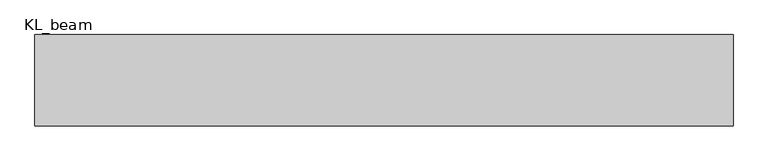
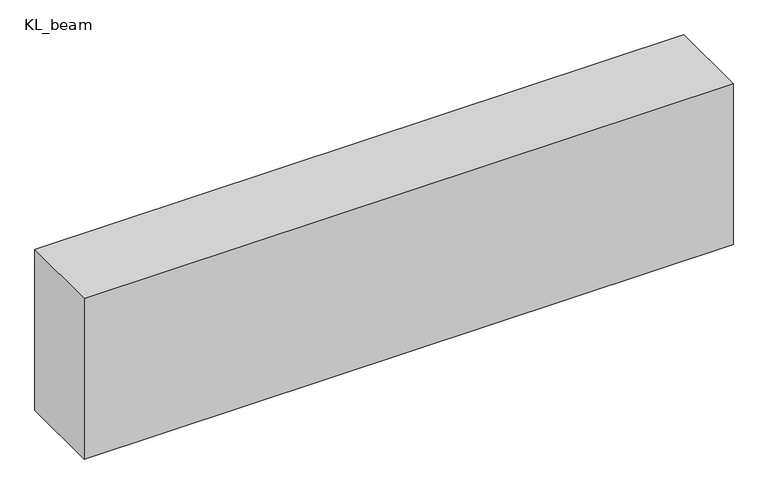
"""IFC4 building model written with IfcOpenShell, lengths in millimetres: beam geometry, 混凝土 - 矩形梁 : KL_beam."""

import ifcopenshell
import ifcopenshell.guid

model = None  # the IFC model being written
_history = None  # IfcOwnerHistory: only IFC2X3 demands one
_inside = {}  # id of a spatial element -> (the spatial element, [elements in it])
_under = {}  # id of a project, library or spatial element -> (it, [spatial elements below it])
_declared = {}  # id of a project -> (the project, [libraries it declares])
_typed = {}  # id of a type object -> (the type object, [elements of that type])
_made_of = {}  # id of a material, layer set ... -> (it, [elements and type objects made of it])


def new_model(schema):
    """Start an empty IFC model of exactly this schema.

    Asked for "IFC4X3", IfcOpenShell would pick the latest addendum, in which some entities
    have other attributes; the version numbers below select the first issue.
    IFC2X3 requires an IfcOwnerHistory on every rooted entity: one is made here for all.
    """
    global model, _history
    if schema == "IFC4X3":
        model = ifcopenshell.file(schema_version=(4, 3, 0, 0))
    else:
        model = ifcopenshell.file(schema=schema)
    _inside.clear()
    _under.clear()
    _declared.clear()
    _typed.clear()
    _made_of.clear()
    _history = None
    if model.schema == "IFC2X3":
        org = make("IfcOrganization", Name="unknown")
        user = make(
            "IfcPersonAndOrganization",
            ThePerson=make("IfcPerson", FamilyName="unknown"),
            TheOrganization=org,
        )
        app = make(
            "IfcApplication",
            ApplicationDeveloper=org,
            Version="unknown",
            ApplicationFullName="unknown",
            ApplicationIdentifier="unknown",
        )
        _history = make(
            "IfcOwnerHistory",
            OwningUser=user,
            OwningApplication=app,
            ChangeAction="ADDED",
            CreationDate=0,
        )
    return model


def make(cls, **values):
    """One entity of the class cls with the attributes given. An attribute that is None is left unset."""
    return model.create_entity(
        cls, **{name: value for name, value in values.items() if value is not None}
    )


def rooted(cls, **values):
    """An entity with a GlobalId (a new one), such as an element, a storey or a relation."""
    return make(cls, GlobalId=ifcopenshell.guid.new(), OwnerHistory=_history, **values)


def si_unit(unit_type, name, prefix=None):
    """IfcSIUnit, for example si_unit("LENGTHUNIT", "METRE", prefix="MILLI")."""
    return make("IfcSIUnit", UnitType=unit_type, Prefix=prefix, Name=name)


def assignment(units):
    """IfcUnitAssignment: the units of a project."""
    return None if units is None else make("IfcUnitAssignment", Units=units)


def point(xyz):
    """IfcCartesianPoint."""
    return None if xyz is None else make("IfcCartesianPoint", Coordinates=xyz)


def direction(xyz):
    """IfcDirection."""
    return None if xyz is None else make("IfcDirection", DirectionRatios=xyz)


def frame(location, z_axis=None, x_axis=None):
    """IfcAxis2Placement3D, a coordinate frame: its origin and axes. An axis left out is left unset."""
    return make(
        "IfcAxis2Placement3D",
        Location=point(location),
        Axis=direction(z_axis),
        RefDirection=direction(x_axis),
    )


def origin():
    """The frame at (0, 0, 0) with its axes left unset."""
    return frame((0.0, 0.0, 0.0))


def place(relative_to, where):
    """IfcLocalPlacement: puts the frame where relative to a parent placement (None: the world)."""
    return make(
        "IfcLocalPlacement", PlacementRelTo=relative_to, RelativePlacement=where
    )


def context(
    kind, dimensions, precision=None, world=None, true_north=None, identifier=None
):
    """IfcGeometricRepresentationContext, for example the 3D "Model" context."""
    return make(
        "IfcGeometricRepresentationContext",
        ContextIdentifier=identifier,
        ContextType=kind,
        CoordinateSpaceDimension=dimensions,
        Precision=precision,
        WorldCoordinateSystem=world,
        TrueNorth=true_north,
    )


def project(units=None, contexts=None):
    """IfcProject with its units and contexts."""
    return rooted(
        "IfcProject",
        Name="project",
        RepresentationContexts=contexts,
        UnitsInContext=assignment(units),
    )


def spatial(cls, under=None, at=None, **own):
    """A site, building, storey or space (cls), placed at a placement, below another one or the project."""
    s = rooted(cls, ObjectPlacement=at, **own)
    if under is not None:
        _under.setdefault(under.id(), (under, []))[1].append(s)
    return s


def polyline(points):
    """IfcPolyline through the points."""
    return make("IfcPolyline", Points=[point(p) for p in points])


def outline(outer, holes=None, kind="AREA"):
    """IfcArbitraryClosedProfileDef: a profile drawn as a closed curve; with holes, ...WithVoids."""
    if holes is None:
        return make("IfcArbitraryClosedProfileDef", ProfileType=kind, OuterCurve=outer)
    return make(
        "IfcArbitraryProfileDefWithVoids",
        ProfileType=kind,
        OuterCurve=outer,
        InnerCurves=holes,
    )


def extrude(swept, where, along, depth):
    """IfcExtrudedAreaSolid: the profile swept, set in the frame where, extruded along a direction by depth."""
    return make(
        "IfcExtrudedAreaSolid",
        SweptArea=swept,
        Position=where,
        ExtrudedDirection=direction(along),
        Depth=depth,
    )


def shape(context_of_items, identifier, shape_type, items):
    """IfcShapeRepresentation: the items that make up one representation, for example the "Body"."""
    return make(
        "IfcShapeRepresentation",
        ContextOfItems=context_of_items,
        RepresentationIdentifier=identifier,
        RepresentationType=shape_type,
        Items=items,
    )


def source(mapping_origin, context_of_items, identifier, shape_type, items):
    """IfcRepresentationMap: a shape defined once, which mapped items show again and again."""
    return make(
        "IfcRepresentationMap",
        MappingOrigin=mapping_origin,
        MappedRepresentation=shape(context_of_items, identifier, shape_type, items),
    )


def transform(
    local_origin,
    x_axis=None,
    y_axis=None,
    z_axis=None,
    scale=None,
    scale2=None,
    scale3=None,
    uniform=True,
):
    """IfcCartesianTransformationOperator3D, or its non-uniform kind. x_axis, y_axis, z_axis: its Axis1, 2, 3."""
    if uniform:
        return make(
            "IfcCartesianTransformationOperator3D",
            Axis1=direction(x_axis),
            Axis2=direction(y_axis),
            LocalOrigin=point(local_origin),
            Scale=scale,
            Axis3=direction(z_axis),
        )
    return make(
        "IfcCartesianTransformationOperator3DnonUniform",
        Axis1=direction(x_axis),
        Axis2=direction(y_axis),
        LocalOrigin=point(local_origin),
        Scale=scale,
        Axis3=direction(z_axis),
        Scale2=scale2,
        Scale3=scale3,
    )


def mapped(mapping_source, mapping_target):
    """IfcMappedItem: shows the shape of a source again, moved by a transform."""
    return make(
        "IfcMappedItem", MappingSource=mapping_source, MappingTarget=mapping_target
    )


def made_of(thing, what):
    """Note that an element or type object is made of a material, layer set ...; save() writes the relation."""
    if what is not None:
        _made_of.setdefault(what.id(), (what, []))[1].append(thing)
    return thing


def element(
    cls,
    number,
    at=None,
    inside=None,
    cuts=None,
    type_object=None,
    material=None,
    context=None,
    identifier="Body",
    shape_type=None,
    held_by="IfcProductDefinitionShape",
    body=None,
    shapes=None,
    **own,
):
    """One element of the class cls, such as IfcWall. Its Tag is "e" and its number.

    at: its placement. inside: the storey or other place that contains it. cuts: it is an
    opening in that element (IfcRelVoidsElement). A single representation is given by context,
    identifier, shape_type and body (its items); several are given by shapes. held_by: the class
    of the entity that holds the representations. save() writes the other relations.
    """
    e = rooted(cls, Tag="e%d" % number, ObjectPlacement=at, **own)
    if body is not None:
        shapes = [shape(context, identifier, shape_type, body)]
    if shapes is not None:
        e.Representation = make(held_by, Representations=shapes)
    if inside is not None:
        _inside.setdefault(inside.id(), (inside, []))[1].append(e)
    if cuts is not None:
        rooted(
            "IfcRelVoidsElement", RelatingBuildingElement=cuts, RelatedOpeningElement=e
        )
    if type_object is not None:
        _typed.setdefault(type_object.id(), (type_object, []))[1].append(e)
    return made_of(e, material)


def aggregate(whole, parts):
    """IfcRelAggregates: a whole, such as a stair, and the parts it consists of."""
    return rooted("IfcRelAggregates", RelatingObject=whole, RelatedObjects=parts)


def save(model, path):
    """Write the relations noted so far, then the file.

    IfcRelAggregates (storeys below a building ...), IfcRelContainedInSpatialStructure (elements
    in a storey), IfcRelDefinesByType, IfcRelAssociatesMaterial and IfcRelDeclares: one each for
    every whole, place, type object, material and project.
    """
    for whole, parts in _under.values():
        aggregate(whole, parts)
    for where, things in _inside.values():
        rooted(
            "IfcRelContainedInSpatialStructure",
            RelatedElements=things,
            RelatingStructure=where,
        )
    for kind, things in _typed.values():
        rooted("IfcRelDefinesByType", RelatedObjects=things, RelatingType=kind)
    for what, things in _made_of.values():
        rooted("IfcRelAssociatesMaterial", RelatedObjects=things, RelatingMaterial=what)
    for by, libraries in _declared.values():
        rooted("IfcRelDeclares", RelatingContext=by, RelatedDefinitions=libraries)
    model.write(path)


def kl_beam_252f1571(model_context):
    return source(origin(), model_context, "Body", "SweptSolid", [
        extrude(outline(polyline([(1526.0, 200.0), (1526.0, -200.0), (-1526.0, -200.0), (-1526.0, 200.0), (1526.0, 200.0)])), frame((0.0, 0.0, -400.0), z_axis=(0.0, 0.0, 1.0), x_axis=(1.0, 0.0, 0.0)), (0.0, 0.0, 1.0), 800.0),
    ])


if __name__ == "__main__":
    model = new_model("IFC4")
    model_context = context("Model", 3, world=origin())
    ifc_project = project(units=[si_unit("LENGTHUNIT", "METRE", prefix="MILLI")], contexts=[model_context])
    site = spatial("IfcSite", under=ifc_project)
    building = spatial("IfcBuilding", under=site)
    placement = place(None, origin())
    kl_beam_shape = kl_beam_252f1571(model_context)
    element("IfcBeam", 1, ObjectType="混凝土 - 矩形梁 : KL_beam", at=placement, inside=building, context=model_context, shape_type="MappedRepresentation", body=[
        mapped(kl_beam_shape, transform((0.0, 0.0, 0.0), x_axis=(1.0, 0.0, 0.0), y_axis=(0.0, 1.0, 0.0), z_axis=(0.0, 0.0, 1.0))),
    ])
    save(model, "model.ifc")

# Revit data of these elements
# Type "混凝土 - 矩形梁 : KL_beam"
#   Length [instance default] = 1524 mm
#   b = 400 mm
#   h = 800 mm
#   Structural Material [instance default] = 混凝土 - 现场浇注混凝土
#   Assembly Code = ""
# Element 1 (IfcBeam, "混凝土 - 矩形梁 : KL_beam")
#   Structural Material = none
# Materials
#   "混凝土 - 现场浇注混凝土": class "混凝土", colour RGB 192 192 192, transparency 0
